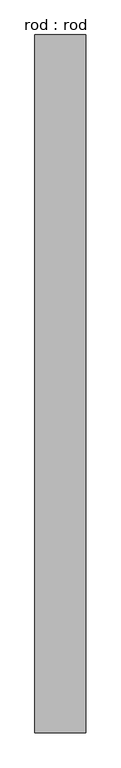
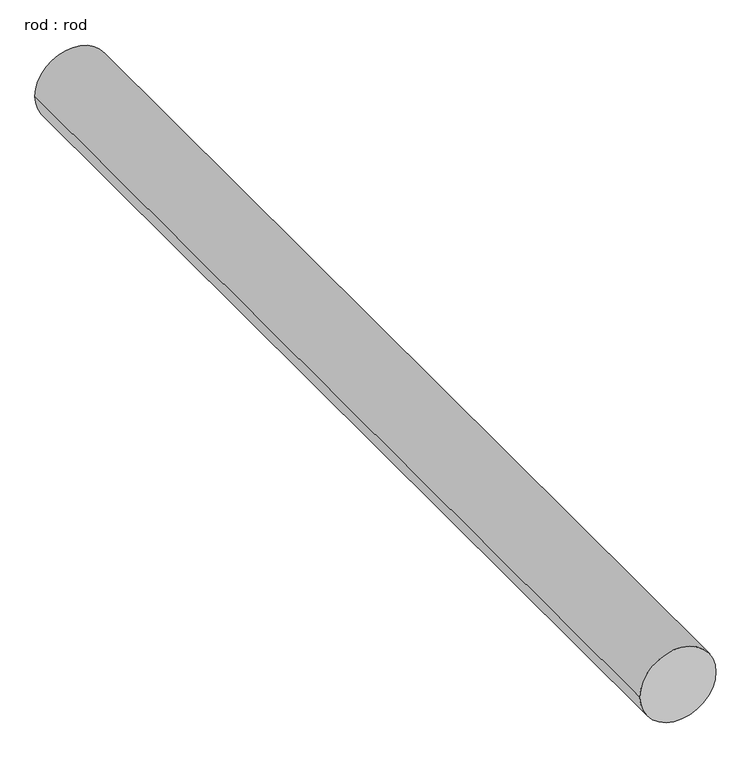
"""IFC4 building model written with IfcOpenShell, lengths in millimetres: proxy geometry, rod : rod."""

from ifc_helpers import new_model, si_unit, point, frame, frame_2d, origin, place, context, project, spatial, circle_curve, trimmed, segment, composite_curve, outline, extrude, source, transform, mapped, element, save


def rod_rod_e43c47ca(model_context):
    return source(origin(), model_context, "Body", "SweptSolid", [
        extrude(outline(composite_curve([segment(trimmed(circle_curve(frame_2d((0.0108462, 0.0)), 200.0), [point((0.0108462, 200.0))], [point((0.0108462, -200.0))], False, "CARTESIAN"), True, "CONTINUOUS"), segment(trimmed(circle_curve(frame_2d((0.0108462, 0.0)), 200.0), [point((0.0108462, -200.0))], [point((0.0108462, 200.0))], False, "CARTESIAN"), True, "CONTINUOUS")], self_intersect=False)), frame((0.0, 1341.6887551, 0.0), z_axis=(0.0, 1.0, 0.0), x_axis=(0.0, 0.0, 1.0)), (0.0, 0.0, 1.0), 5502.0797204),
    ])


if __name__ == "__main__":
    model = new_model("IFC4")
    model_context = context("Model", 3, world=origin())
    ifc_project = project(units=[si_unit("LENGTHUNIT", "METRE", prefix="MILLI")], contexts=[model_context])
    site = spatial("IfcSite", under=ifc_project)
    building = spatial("IfcBuilding", under=site)
    placement = place(None, origin())
    rod_rod_shape = rod_rod_e43c47ca(model_context)
    element("IfcBuildingElementProxy", 1, Name="rod : rod", ObjectType="rod : rod", at=placement, inside=building, context=model_context, shape_type="MappedRepresentation", body=[
        mapped(rod_rod_shape, transform((0.0, 0.0, 0.0), x_axis=(1.0, 0.0, 0.0), y_axis=(0.0, 1.0, 0.0), z_axis=(0.0, 0.0, 1.0))),
    ])
    save(model, "model.ifc")

# Revit data of these elements
# Type "rod : rod"
#   Default Elevation = 0
